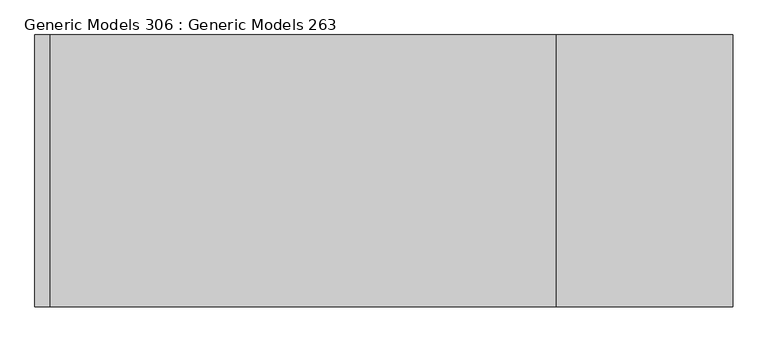
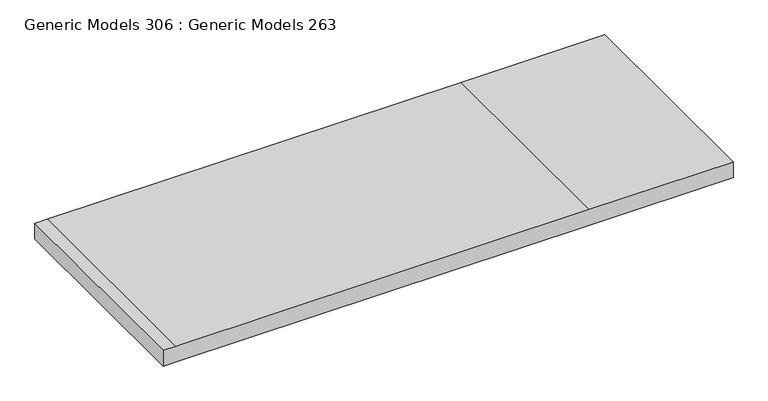
"""IFC4 building model written with IfcOpenShell, lengths in millimetres: proxy geometry, Generic Models 306 : Generic Models 263."""

from ifc_helpers import new_model, si_unit, point, frame, frame_2d, origin, place, context, project, spatial, polyline, circle_curve, trimmed, segment, composite_curve, outline, extrude, source, transform, mapped, element, save


def generic_models_306_generic_models_263_110f4e42(model_context):
    return source(origin(), model_context, "Body", "SweptSolid", [
        extrude(outline(composite_curve([segment(polyline([(-304.9836851, 64122.5797726), (-304.9836851, 63653.8340403), (-914.0337686, 63653.8340403), (-914.0337686, 64148.9956464)]), True, "CONTINUOUS"), segment(trimmed(circle_curve(frame_2d((-219607.3320282, 71742.5797726)), 218825.0927648), [point((-914.0337686, 64148.9956464))], [point((-914.5836851, 79351.9848532))], True, "CARTESIAN"), True, "CONTINUOUS"), segment(polyline([(-914.5836851, 79351.9848532), (-914.5836851, 84681.146689), (-304.9836851, 84681.146689), (-304.9836851, 79362.5797726)]), True, "CONTINUOUS"), segment(trimmed(circle_curve(frame_2d((-219607.3320282, 71742.5797726)), 219434.6927648), [point((-304.9836851, 79362.5797726))], [point((-304.9836851, 64122.5797726))], False, "CARTESIAN"), True, "CONTINUOUS")], self_intersect=False)), frame((0.0, -3202.6200333, 0.0), z_axis=(0.0, 1.0, 0.0), x_axis=(0.0, 0.0, 1.0)), (0.0, 0.0, 1.0), 8183.6367002),
    ])


if __name__ == "__main__":
    model = new_model("IFC4")
    model_context = context("Model", 3, world=origin())
    ifc_project = project(units=[si_unit("LENGTHUNIT", "METRE", prefix="MILLI")], contexts=[model_context])
    site = spatial("IfcSite", under=ifc_project)
    building = spatial("IfcBuilding", under=site)
    placement = place(None, origin())
    generic_models_306_generic_models_263_shape = generic_models_306_generic_models_263_110f4e42(model_context)
    element("IfcBuildingElementProxy", 1, Name="Generic Models 306 : Generic Models 263", ObjectType="Generic Models 306 : Generic Models 263", at=placement, inside=building, context=model_context, shape_type="MappedRepresentation", body=[
        mapped(generic_models_306_generic_models_263_shape, transform((0.0, 0.0, 0.0), x_axis=(1.0, 0.0, 0.0), y_axis=(0.0, 1.0, 0.0), z_axis=(0.0, 0.0, 1.0))),
    ])
    save(model, "model.ifc")

# Revit data of these elements
# Element 1 (IfcBuildingElementProxy, "Generic Models 306 : Generic Models 263")
#   Materials on its faces: "EXISTING GRADE"
# Materials
#   "EXISTING GRADE": class "Miscellaneous", colour RGB 128 97 77, transparency 0, Cost = 0
